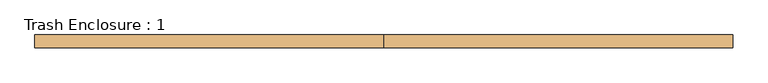
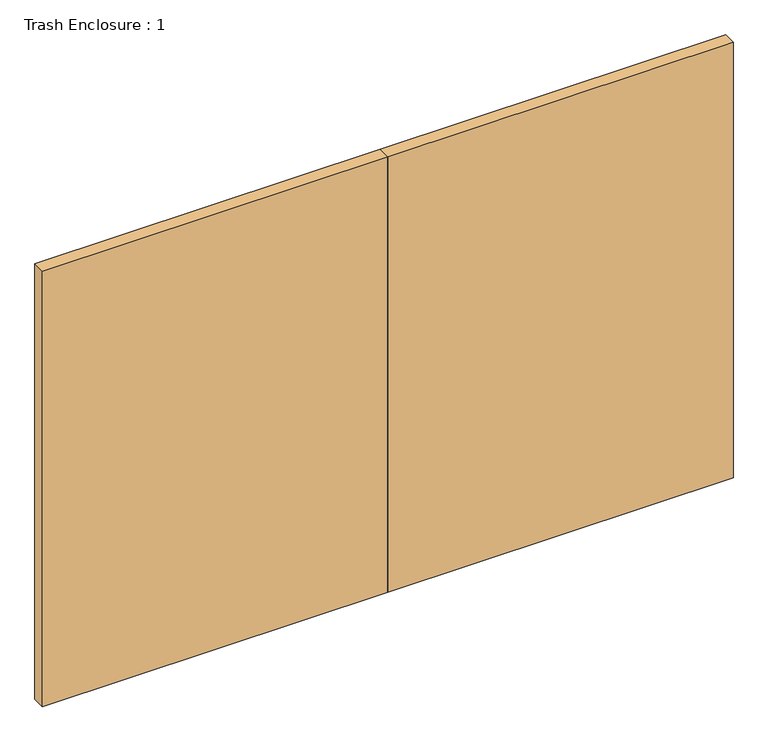
"""IFC4 building model written with IfcOpenShell, lengths in millimetres: door geometry, Trash Enclosure : 1."""

import ifcopenshell
import ifcopenshell.guid

model = None  # the IFC model being written
_history = None  # IfcOwnerHistory: only IFC2X3 demands one
_inside = {}  # id of a spatial element -> (the spatial element, [elements in it])
_under = {}  # id of a project, library or spatial element -> (it, [spatial elements below it])
_declared = {}  # id of a project -> (the project, [libraries it declares])
_typed = {}  # id of a type object -> (the type object, [elements of that type])
_made_of = {}  # id of a material, layer set ... -> (it, [elements and type objects made of it])


def new_model(schema):
    """Start an empty IFC model of exactly this schema.

    Asked for "IFC4X3", IfcOpenShell would pick the latest addendum, in which some entities
    have other attributes; the version numbers below select the first issue.
    IFC2X3 requires an IfcOwnerHistory on every rooted entity: one is made here for all.
    """
    global model, _history
    if schema == "IFC4X3":
        model = ifcopenshell.file(schema_version=(4, 3, 0, 0))
    else:
        model = ifcopenshell.file(schema=schema)
    _inside.clear()
    _under.clear()
    _declared.clear()
    _typed.clear()
    _made_of.clear()
    _history = None
    if model.schema == "IFC2X3":
        org = make("IfcOrganization", Name="unknown")
        user = make(
            "IfcPersonAndOrganization",
            ThePerson=make("IfcPerson", FamilyName="unknown"),
            TheOrganization=org,
        )
        app = make(
            "IfcApplication",
            ApplicationDeveloper=org,
            Version="unknown",
            ApplicationFullName="unknown",
            ApplicationIdentifier="unknown",
        )
        _history = make(
            "IfcOwnerHistory",
            OwningUser=user,
            OwningApplication=app,
            ChangeAction="ADDED",
            CreationDate=0,
        )
    return model


def make(cls, **values):
    """One entity of the class cls with the attributes given. An attribute that is None is left unset."""
    return model.create_entity(
        cls, **{name: value for name, value in values.items() if value is not None}
    )


def rooted(cls, **values):
    """An entity with a GlobalId (a new one), such as an element, a storey or a relation."""
    return make(cls, GlobalId=ifcopenshell.guid.new(), OwnerHistory=_history, **values)


def si_unit(unit_type, name, prefix=None):
    """IfcSIUnit, for example si_unit("LENGTHUNIT", "METRE", prefix="MILLI")."""
    return make("IfcSIUnit", UnitType=unit_type, Prefix=prefix, Name=name)


def assignment(units):
    """IfcUnitAssignment: the units of a project."""
    return None if units is None else make("IfcUnitAssignment", Units=units)


def point(xyz):
    """IfcCartesianPoint."""
    return None if xyz is None else make("IfcCartesianPoint", Coordinates=xyz)


def direction(xyz):
    """IfcDirection."""
    return None if xyz is None else make("IfcDirection", DirectionRatios=xyz)


def frame(location, z_axis=None, x_axis=None):
    """IfcAxis2Placement3D, a coordinate frame: its origin and axes. An axis left out is left unset."""
    return make(
        "IfcAxis2Placement3D",
        Location=point(location),
        Axis=direction(z_axis),
        RefDirection=direction(x_axis),
    )


def origin():
    """The frame at (0, 0, 0) with its axes left unset."""
    return frame((0.0, 0.0, 0.0))


def origin_with_axes():
    """The frame at (0, 0, 0) with the z axis (0, 0, 1) and the x axis (1, 0, 0) written out."""
    return frame((0.0, 0.0, 0.0), z_axis=(0.0, 0.0, 1.0), x_axis=(1.0, 0.0, 0.0))


def place(relative_to, where):
    """IfcLocalPlacement: puts the frame where relative to a parent placement (None: the world)."""
    return make(
        "IfcLocalPlacement", PlacementRelTo=relative_to, RelativePlacement=where
    )


def context(
    kind, dimensions, precision=None, world=None, true_north=None, identifier=None
):
    """IfcGeometricRepresentationContext, for example the 3D "Model" context."""
    return make(
        "IfcGeometricRepresentationContext",
        ContextIdentifier=identifier,
        ContextType=kind,
        CoordinateSpaceDimension=dimensions,
        Precision=precision,
        WorldCoordinateSystem=world,
        TrueNorth=true_north,
    )


def project(units=None, contexts=None):
    """IfcProject with its units and contexts."""
    return rooted(
        "IfcProject",
        Name="project",
        RepresentationContexts=contexts,
        UnitsInContext=assignment(units),
    )


def spatial(cls, under=None, at=None, **own):
    """A site, building, storey or space (cls), placed at a placement, below another one or the project."""
    s = rooted(cls, ObjectPlacement=at, **own)
    if under is not None:
        _under.setdefault(under.id(), (under, []))[1].append(s)
    return s


def polyline(points):
    """IfcPolyline through the points."""
    return make("IfcPolyline", Points=[point(p) for p in points])


def outline(outer, holes=None, kind="AREA"):
    """IfcArbitraryClosedProfileDef: a profile drawn as a closed curve; with holes, ...WithVoids."""
    if holes is None:
        return make("IfcArbitraryClosedProfileDef", ProfileType=kind, OuterCurve=outer)
    return make(
        "IfcArbitraryProfileDefWithVoids",
        ProfileType=kind,
        OuterCurve=outer,
        InnerCurves=holes,
    )


def extrude(swept, where, along, depth):
    """IfcExtrudedAreaSolid: the profile swept, set in the frame where, extruded along a direction by depth."""
    return make(
        "IfcExtrudedAreaSolid",
        SweptArea=swept,
        Position=where,
        ExtrudedDirection=direction(along),
        Depth=depth,
    )


def shape(context_of_items, identifier, shape_type, items):
    """IfcShapeRepresentation: the items that make up one representation, for example the "Body"."""
    return make(
        "IfcShapeRepresentation",
        ContextOfItems=context_of_items,
        RepresentationIdentifier=identifier,
        RepresentationType=shape_type,
        Items=items,
    )


def source(mapping_origin, context_of_items, identifier, shape_type, items):
    """IfcRepresentationMap: a shape defined once, which mapped items show again and again."""
    return make(
        "IfcRepresentationMap",
        MappingOrigin=mapping_origin,
        MappedRepresentation=shape(context_of_items, identifier, shape_type, items),
    )


def transform(
    local_origin,
    x_axis=None,
    y_axis=None,
    z_axis=None,
    scale=None,
    scale2=None,
    scale3=None,
    uniform=True,
):
    """IfcCartesianTransformationOperator3D, or its non-uniform kind. x_axis, y_axis, z_axis: its Axis1, 2, 3."""
    if uniform:
        return make(
            "IfcCartesianTransformationOperator3D",
            Axis1=direction(x_axis),
            Axis2=direction(y_axis),
            LocalOrigin=point(local_origin),
            Scale=scale,
            Axis3=direction(z_axis),
        )
    return make(
        "IfcCartesianTransformationOperator3DnonUniform",
        Axis1=direction(x_axis),
        Axis2=direction(y_axis),
        LocalOrigin=point(local_origin),
        Scale=scale,
        Axis3=direction(z_axis),
        Scale2=scale2,
        Scale3=scale3,
    )


def mapped(mapping_source, mapping_target):
    """IfcMappedItem: shows the shape of a source again, moved by a transform."""
    return make(
        "IfcMappedItem", MappingSource=mapping_source, MappingTarget=mapping_target
    )


def made_of(thing, what):
    """Note that an element or type object is made of a material, layer set ...; save() writes the relation."""
    if what is not None:
        _made_of.setdefault(what.id(), (what, []))[1].append(thing)
    return thing


def element(
    cls,
    number,
    at=None,
    inside=None,
    cuts=None,
    type_object=None,
    material=None,
    context=None,
    identifier="Body",
    shape_type=None,
    held_by="IfcProductDefinitionShape",
    body=None,
    shapes=None,
    **own,
):
    """One element of the class cls, such as IfcWall. Its Tag is "e" and its number.

    at: its placement. inside: the storey or other place that contains it. cuts: it is an
    opening in that element (IfcRelVoidsElement). A single representation is given by context,
    identifier, shape_type and body (its items); several are given by shapes. held_by: the class
    of the entity that holds the representations. save() writes the other relations.
    """
    e = rooted(cls, Tag="e%d" % number, ObjectPlacement=at, **own)
    if body is not None:
        shapes = [shape(context, identifier, shape_type, body)]
    if shapes is not None:
        e.Representation = make(held_by, Representations=shapes)
    if inside is not None:
        _inside.setdefault(inside.id(), (inside, []))[1].append(e)
    if cuts is not None:
        rooted(
            "IfcRelVoidsElement", RelatingBuildingElement=cuts, RelatedOpeningElement=e
        )
    if type_object is not None:
        _typed.setdefault(type_object.id(), (type_object, []))[1].append(e)
    return made_of(e, material)


def aggregate(whole, parts):
    """IfcRelAggregates: a whole, such as a stair, and the parts it consists of."""
    return rooted("IfcRelAggregates", RelatingObject=whole, RelatedObjects=parts)


def save(model, path):
    """Write the relations noted so far, then the file.

    IfcRelAggregates (storeys below a building ...), IfcRelContainedInSpatialStructure (elements
    in a storey), IfcRelDefinesByType, IfcRelAssociatesMaterial and IfcRelDeclares: one each for
    every whole, place, type object, material and project.
    """
    for whole, parts in _under.values():
        aggregate(whole, parts)
    for where, things in _inside.values():
        rooted(
            "IfcRelContainedInSpatialStructure",
            RelatedElements=things,
            RelatingStructure=where,
        )
    for kind, things in _typed.values():
        rooted("IfcRelDefinesByType", RelatedObjects=things, RelatingType=kind)
    for what, things in _made_of.values():
        rooted("IfcRelAssociatesMaterial", RelatedObjects=things, RelatingMaterial=what)
    for by, libraries in _declared.values():
        rooted("IfcRelDeclares", RelatingContext=by, RelatedDefinitions=libraries)
    model.write(path)


def trash_enclosure_1_93c10759(model_context):
    return source(origin(), model_context, "Body", "SweptSolid", [
        extrude(outline(polyline([(0.0, 50.8), (1371.6, 50.8), (1371.6, 0.0), (0.0, 0.0), (0.0, 50.8)])), origin_with_axes(), (0.0, 0.0, 1.0), 1828.8),
        extrude(outline(polyline([(-1371.6, 50.8), (0.0, 50.8), (0.0, 0.0), (-1371.6, 0.0), (-1371.6, 50.8)])), origin_with_axes(), (0.0, 0.0, 1.0), 1828.8),
    ])


if __name__ == "__main__":
    model = new_model("IFC4")
    model_context = context("Model", 3, world=origin())
    ifc_project = project(units=[si_unit("LENGTHUNIT", "METRE", prefix="MILLI")], contexts=[model_context])
    site = spatial("IfcSite", under=ifc_project)
    building = spatial("IfcBuilding", under=site)
    placement = place(None, origin())
    trash_enclosure_1_shape = trash_enclosure_1_93c10759(model_context)
    element("IfcDoor", 1, ObjectType="Trash Enclosure : 1", at=placement, inside=building, context=model_context, shape_type="MappedRepresentation", body=[
        mapped(trash_enclosure_1_shape, transform((0.0, 0.0, 0.0), x_axis=(1.0, 0.0, 0.0), y_axis=(0.0, 1.0, 0.0), z_axis=(0.0, 0.0, 1.0))),
    ])
    save(model, "model.ifc")

# Revit data of these elements
# Type "Trash Enclosure : 1"
#   Type Mark = "33"
#   Construction Type Id = "DOOR"
#   Assembly Code = "C1020"
#   Analytic Construction = "Wooden"
#   Thickness = 0' - 2"
#   Thermal Resistance (R) = 0.455703 (m²·K)/W
#   Swing Angle [instance default] = 90.00°
#   Panel Width = 4' - 6"
#   Heat Transfer Coefficient (U) = 2.19465 W/(m²·K)
#   Height = 6' - 0"
#   Trim Projection Ext = 0' - 1"
#   Trim Projection Int = 0' - 1"
#   Trim Width = 0' - 3"
#   Width = 9' - 0"
#   Panel Material = CORRUGATED ALUMINIUM PANELS (TO MATCH THOSE ON MAIN BUILDING)
#   Trim Material = CORRUGATED ALUMINIUM PANELS (TO MATCH THOSE ON MAIN BUILDING)
#   Visual Light Transmittance = 0
#   Solar Heat Gain Coefficient = 0
#   Function = (empty or 0)
#   Wall Closure = (empty or 0)
# Element 1 (IfcDoor, "Trash Enclosure : 1")
#   Materials on its faces: "CORRUGATED ALUMINIUM PANELS (TO MATCH THOSE ON MAIN BUILDING)"
# Materials
#   "CORRUGATED ALUMINIUM PANELS (TO MATCH THOSE ON MAIN BUILDING)": class "Generic", colour RGB 108 108 108, transparency 0, Cost = 0
